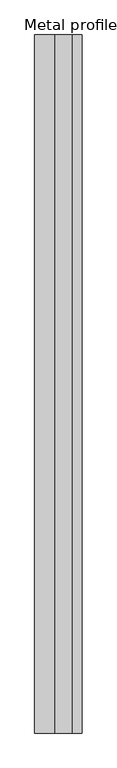
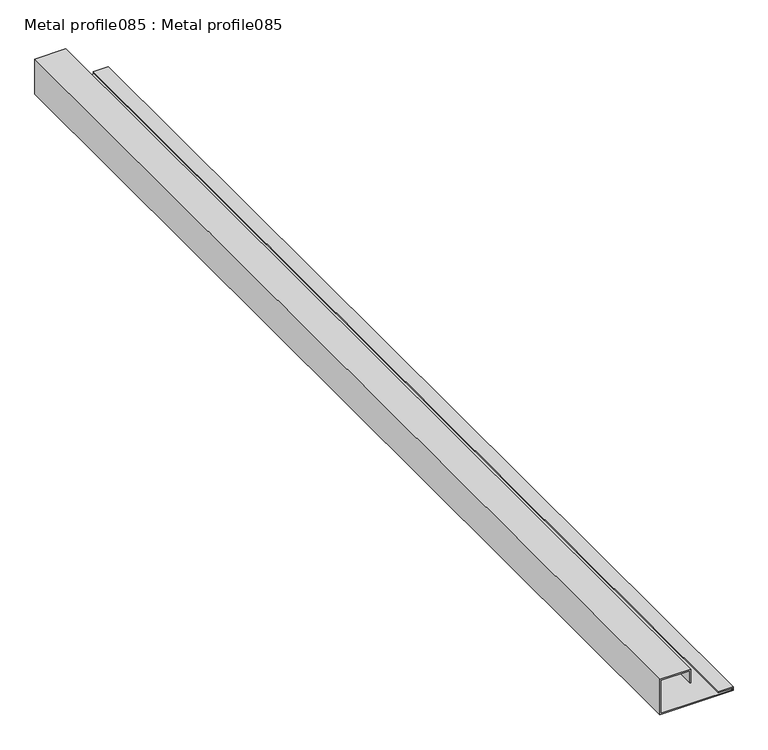
"""IFC4 building model written with IfcOpenShell, lengths in millimetres: proxy geometry, Metal profile085 : Metal profile085."""

from ifc_helpers import new_model, si_unit, frame, origin, place, context, project, spatial, polyline, outline, extrude, source, transform, mapped, element, save


def metal_profile085_metal_profile085_73fac49b(model_context):
    return source(origin(), model_context, "Body", "SweptSolid", [
        extrude(outline(polyline([(42529.5797448, -2355.870033), (42529.5797448, -2330.1068494), (42526.7125573, -2330.1068494), (42526.7125573, -2461.7059705), (42591.4859948, -2461.7059705), (42591.4859948, -2408.3607556), (42567.3922448, -2408.3607556), (42567.3922448, -2406.3607556), (42593.4859948, -2406.3607556), (42593.4859948, -2463.7059705), (42524.7125573, -2463.7059705), (42524.7125573, -2328.1068494), (42531.5797448, -2328.1068494), (42531.5797448, -2355.870033), (42529.5797448, -2355.870033)])), frame((0.0, -1052.8906574, 0.0), z_axis=(0.0, 1.0, 0.0), x_axis=(0.0, 0.0, 1.0)), (0.0, 0.0, 1.0), 2000.0),
    ])


if __name__ == "__main__":
    model = new_model("IFC4")
    model_context = context("Model", 3, world=origin())
    ifc_project = project(units=[si_unit("LENGTHUNIT", "METRE", prefix="MILLI")], contexts=[model_context])
    site = spatial("IfcSite", under=ifc_project)
    building = spatial("IfcBuilding", under=site)
    placement = place(None, origin())
    metal_profile085_metal_profile085_shape = metal_profile085_metal_profile085_73fac49b(model_context)
    element("IfcBuildingElementProxy", 1, Name="Metal profile085 : Metal profile085", ObjectType="Metal profile085 : Metal profile085", at=placement, inside=building, context=model_context, shape_type="MappedRepresentation", body=[
        mapped(metal_profile085_metal_profile085_shape, transform((0.0, 0.0, 0.0), x_axis=(1.0, 0.0, 0.0), y_axis=(0.0, 1.0, 0.0), z_axis=(0.0, 0.0, 1.0))),
    ])
    save(model, "model.ifc")

# Revit data of these elements
# Type "Metal profile085 : Metal profile085"
#   NameOverride = "Metal profile085"
# Element 1 (IfcBuildingElementProxy, "Metal profile085 : Metal profile085")
#   Materials on its faces: "RECEIVER TRIM 1393"
# Materials
#   "RECEIVER TRIM 1393": class "Unassigned", colour RGB 255 250 0, transparency 0
